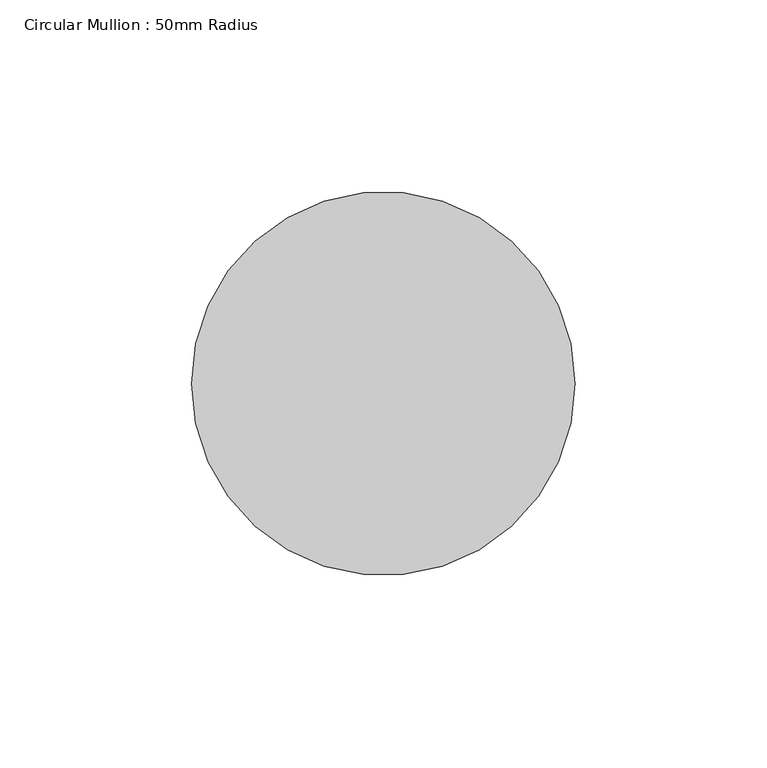
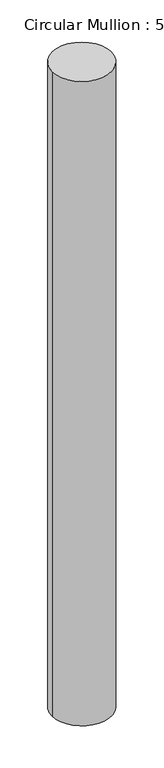
"""IFC4 building model written with IfcOpenShell, lengths in millimetres: member geometry, Circular Mullion : 50mm Radius."""

from ifc_helpers import new_model, si_unit, point, frame, origin, origin_2d, place, context, project, spatial, circle_curve, trimmed, segment, composite_curve, outline, extrude, source, transform, mapped, element, save


def circular_mullion_50mm_radius_05651e4f(model_context):
    return source(origin(), model_context, "Body", "SweptSolid", [
        extrude(outline(composite_curve([segment(trimmed(circle_curve(origin_2d(), 50.0), [point((50.0, 0.0))], [point((-50.0, 0.0))], False, "CARTESIAN"), True, "CONTINUOUS"), segment(trimmed(circle_curve(origin_2d(), 50.0), [point((-50.0, 0.0))], [point((50.0, 0.0))], False, "CARTESIAN"), True, "CONTINUOUS")], self_intersect=False)), frame((0.0, 0.0, -1147.058332), z_axis=(0.0, 0.0, 1.0), x_axis=(1.0, 0.0, 0.0)), (0.0, 0.0, 1.0), 1147.058332),
    ])


if __name__ == "__main__":
    model = new_model("IFC4")
    model_context = context("Model", 3, world=origin())
    ifc_project = project(units=[si_unit("LENGTHUNIT", "METRE", prefix="MILLI")], contexts=[model_context])
    site = spatial("IfcSite", under=ifc_project)
    building = spatial("IfcBuilding", under=site)
    placement = place(None, origin())
    circular_mullion_50mm_radius_shape = circular_mullion_50mm_radius_05651e4f(model_context)
    element("IfcMember", 1, ObjectType="Circular Mullion : 50mm Radius", at=placement, inside=building, context=model_context, shape_type="MappedRepresentation", body=[
        mapped(circular_mullion_50mm_radius_shape, transform((0.0, 0.0, 0.0), x_axis=(1.0, 0.0, 0.0), y_axis=(0.0, 1.0, 0.0), z_axis=(0.0, 0.0, 1.0))),
    ])
    save(model, "model.ifc")

# Revit data of these elements
# Type "Circular Mullion : 50mm Radius"
#   built-in parameter 1007350 = 0.164042 (stored number, unit not read)
# Element 1 (IfcMember, "Circular Mullion : 50mm Radius")
#   Materials on its faces: "Aluminium"
# Materials
#   "Aluminium": class "Metal", colour RGB 247 247 247, transparency 0, Description = "Aluminium 6061", Cost = 0
